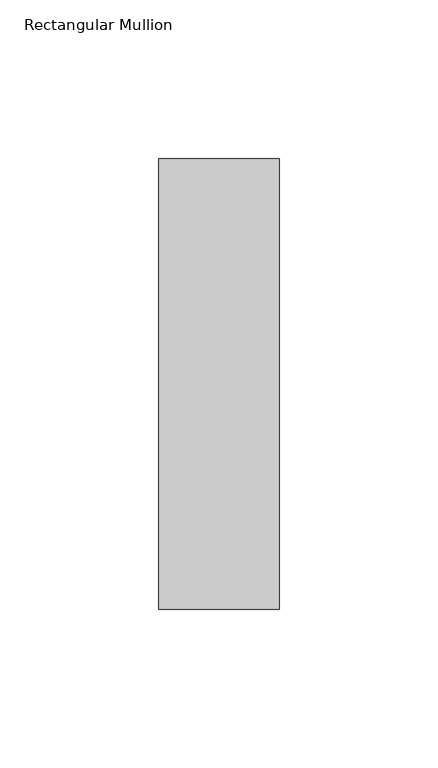
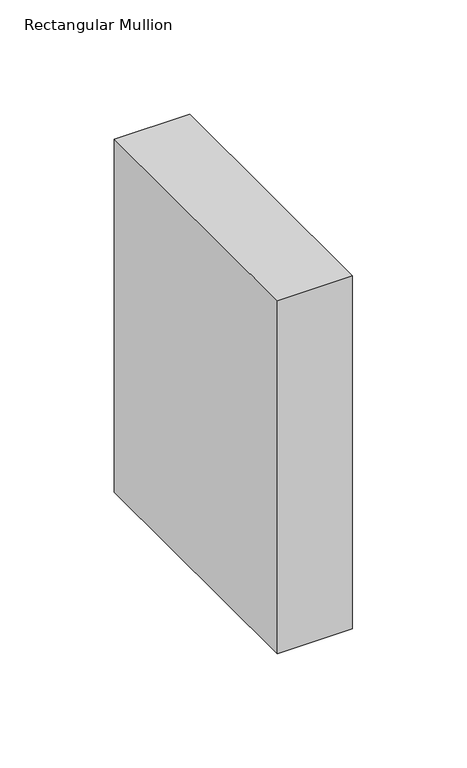
"""IFC4 building model written with IfcOpenShell, lengths in millimetres: member geometry, Rectangular Mullion : NLRS_21_CWM_hsb-regel 38x142_gen_rsf."""

from ifc_helpers import new_model, si_unit, frame, origin, place, context, project, spatial, polyline, outline, extrude, source, transform, mapped, element, save


def rectangular_mullion_45cc79de(model_context):
    return source(origin(), model_context, "Body", "SweptSolid", [
        extrude(outline(polyline([(-38.0, -71.0), (-38.0, 71.0), (0.0, 71.0), (0.0, -71.0), (-38.0, -71.0)])), frame((0.0, 0.0, -188.0000003), z_axis=(0.0, 0.0, 1.0), x_axis=(1.0, 0.0, 0.0)), (0.0, 0.0, 1.0), 188.0000003),
    ])


if __name__ == "__main__":
    model = new_model("IFC4")
    model_context = context("Model", 3, world=origin())
    ifc_project = project(units=[si_unit("LENGTHUNIT", "METRE", prefix="MILLI")], contexts=[model_context])
    site = spatial("IfcSite", under=ifc_project)
    building = spatial("IfcBuilding", under=site)
    placement = place(None, origin())
    rectangular_mullion_shape = rectangular_mullion_45cc79de(model_context)
    element("IfcMember", 1, ObjectType="Rectangular Mullion : NLRS_21_CWM_hsb-regel 38x142_gen_rsf", at=placement, inside=building, context=model_context, shape_type="MappedRepresentation", body=[
        mapped(rectangular_mullion_shape, transform((0.0, 0.0, 0.0), x_axis=(1.0, 0.0, 0.0), y_axis=(0.0, 1.0, 0.0), z_axis=(0.0, 0.0, 1.0))),
    ])
    save(model, "model.ifc")

# Revit data of these elements
# Type "Rectangular Mullion : NLRS_21_CWM_hsb-regel 38x142_gen_rsf"
#   Export Type to IFC As = "IfcWall"
#   Type IfcGUID = "07M7mRoiH1CR8m_RSKIwpF"
#   Assembly Code = "21.10"
#   built-in parameter 1007322 = 0.465879 (stored number, unit not read)
#   built-in parameter 1007321 = 0.062336 (stored number, unit not read)
#   built-in parameter 1007320 = 0.062336 (stored number, unit not read)
# Element 1 (IfcMember, "Rectangular Mullion : NLRS_21_CWM_hsb-regel 38x142_gen_rsf")
#   Materials on its faces: "NLRS_i2_hout naaldhout vuren_gen_rsf"
# Materials
#   "NLRS_i2_hout naaldhout vuren_gen_rsf": class "I - Hout", colour RGB 234 199 147, transparency 0, Keynote = "i2", Manufacturer = "Revit Standards Foundation", URL = "www.revitstandards.org", Description = "hout vuren", Cost = 0
